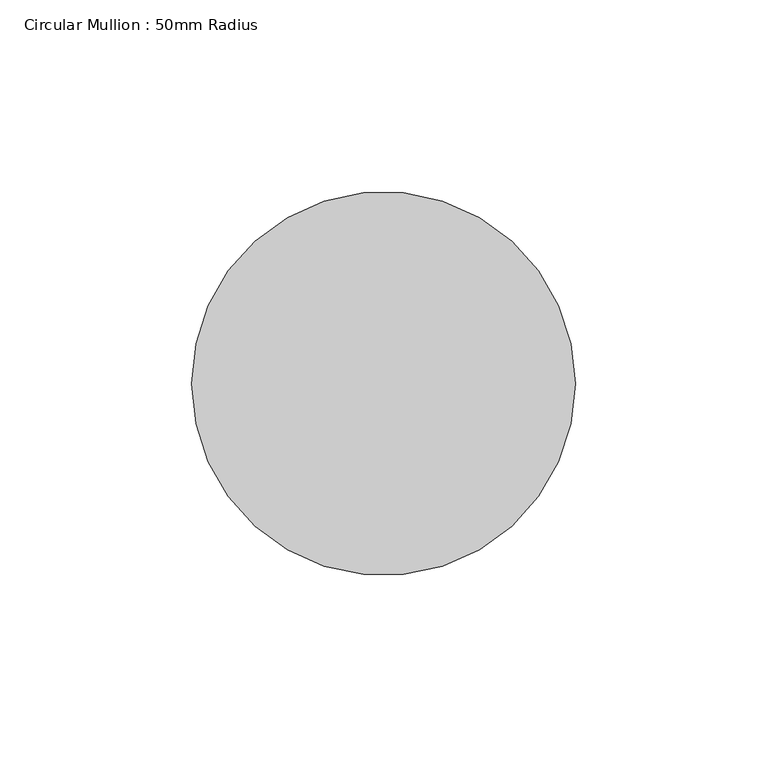
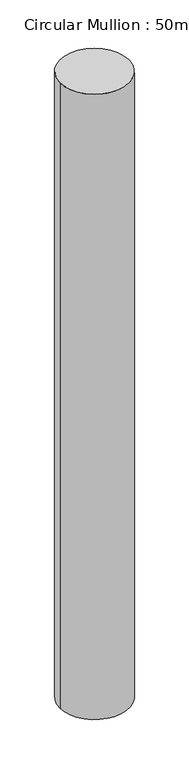
"""IFC4 building model written with IfcOpenShell, lengths in millimetres: member geometry, Circular Mullion : 50mm Radius."""

import ifcopenshell
import ifcopenshell.guid

model = None  # the IFC model being written
_history = None  # IfcOwnerHistory: only IFC2X3 demands one
_inside = {}  # id of a spatial element -> (the spatial element, [elements in it])
_under = {}  # id of a project, library or spatial element -> (it, [spatial elements below it])
_declared = {}  # id of a project -> (the project, [libraries it declares])
_typed = {}  # id of a type object -> (the type object, [elements of that type])
_made_of = {}  # id of a material, layer set ... -> (it, [elements and type objects made of it])


def new_model(schema):
    """Start an empty IFC model of exactly this schema.

    Asked for "IFC4X3", IfcOpenShell would pick the latest addendum, in which some entities
    have other attributes; the version numbers below select the first issue.
    IFC2X3 requires an IfcOwnerHistory on every rooted entity: one is made here for all.
    """
    global model, _history
    if schema == "IFC4X3":
        model = ifcopenshell.file(schema_version=(4, 3, 0, 0))
    else:
        model = ifcopenshell.file(schema=schema)
    _inside.clear()
    _under.clear()
    _declared.clear()
    _typed.clear()
    _made_of.clear()
    _history = None
    if model.schema == "IFC2X3":
        org = make("IfcOrganization", Name="unknown")
        user = make(
            "IfcPersonAndOrganization",
            ThePerson=make("IfcPerson", FamilyName="unknown"),
            TheOrganization=org,
        )
        app = make(
            "IfcApplication",
            ApplicationDeveloper=org,
            Version="unknown",
            ApplicationFullName="unknown",
            ApplicationIdentifier="unknown",
        )
        _history = make(
            "IfcOwnerHistory",
            OwningUser=user,
            OwningApplication=app,
            ChangeAction="ADDED",
            CreationDate=0,
        )
    return model


def make(cls, **values):
    """One entity of the class cls with the attributes given. An attribute that is None is left unset."""
    return model.create_entity(
        cls, **{name: value for name, value in values.items() if value is not None}
    )


def rooted(cls, **values):
    """An entity with a GlobalId (a new one), such as an element, a storey or a relation."""
    return make(cls, GlobalId=ifcopenshell.guid.new(), OwnerHistory=_history, **values)


def si_unit(unit_type, name, prefix=None):
    """IfcSIUnit, for example si_unit("LENGTHUNIT", "METRE", prefix="MILLI")."""
    return make("IfcSIUnit", UnitType=unit_type, Prefix=prefix, Name=name)


def assignment(units):
    """IfcUnitAssignment: the units of a project."""
    return None if units is None else make("IfcUnitAssignment", Units=units)


def point(xyz):
    """IfcCartesianPoint."""
    return None if xyz is None else make("IfcCartesianPoint", Coordinates=xyz)


def direction(xyz):
    """IfcDirection."""
    return None if xyz is None else make("IfcDirection", DirectionRatios=xyz)


def frame(location, z_axis=None, x_axis=None):
    """IfcAxis2Placement3D, a coordinate frame: its origin and axes. An axis left out is left unset."""
    return make(
        "IfcAxis2Placement3D",
        Location=point(location),
        Axis=direction(z_axis),
        RefDirection=direction(x_axis),
    )


def frame_2d(location, x_axis=None):
    """IfcAxis2Placement2D, a coordinate frame in the plane: its origin and x axis."""
    return make(
        "IfcAxis2Placement2D", Location=point(location), RefDirection=direction(x_axis)
    )


def origin():
    """The frame at (0, 0, 0) with its axes left unset."""
    return frame((0.0, 0.0, 0.0))


def origin_2d():
    """The frame at (0, 0) in the plane with its x axis left unset."""
    return frame_2d((0.0, 0.0))


def place(relative_to, where):
    """IfcLocalPlacement: puts the frame where relative to a parent placement (None: the world)."""
    return make(
        "IfcLocalPlacement", PlacementRelTo=relative_to, RelativePlacement=where
    )


def context(
    kind, dimensions, precision=None, world=None, true_north=None, identifier=None
):
    """IfcGeometricRepresentationContext, for example the 3D "Model" context."""
    return make(
        "IfcGeometricRepresentationContext",
        ContextIdentifier=identifier,
        ContextType=kind,
        CoordinateSpaceDimension=dimensions,
        Precision=precision,
        WorldCoordinateSystem=world,
        TrueNorth=true_north,
    )


def project(units=None, contexts=None):
    """IfcProject with its units and contexts."""
    return rooted(
        "IfcProject",
        Name="project",
        RepresentationContexts=contexts,
        UnitsInContext=assignment(units),
    )


def spatial(cls, under=None, at=None, **own):
    """A site, building, storey or space (cls), placed at a placement, below another one or the project."""
    s = rooted(cls, ObjectPlacement=at, **own)
    if under is not None:
        _under.setdefault(under.id(), (under, []))[1].append(s)
    return s


def circle_curve(where, radius):
    """IfcCircle in the frame where."""
    return make("IfcCircle", Position=where, Radius=radius)


def trimmed(basis, trim1, trim2, sense, master):
    """IfcTrimmedCurve: the piece of a basis curve between two trims."""
    return make(
        "IfcTrimmedCurve",
        BasisCurve=basis,
        Trim1=trim1,
        Trim2=trim2,
        SenseAgreement=sense,
        MasterRepresentation=master,
    )


def segment(curve, same_sense, transition):
    """IfcCompositeCurveSegment."""
    return make(
        "IfcCompositeCurveSegment",
        Transition=transition,
        SameSense=same_sense,
        ParentCurve=curve,
    )


def composite_curve(segments, self_intersect=None):
    """IfcCompositeCurve: segments joined end to end."""
    return make("IfcCompositeCurve", Segments=segments, SelfIntersect=self_intersect)


def outline(outer, holes=None, kind="AREA"):
    """IfcArbitraryClosedProfileDef: a profile drawn as a closed curve; with holes, ...WithVoids."""
    if holes is None:
        return make("IfcArbitraryClosedProfileDef", ProfileType=kind, OuterCurve=outer)
    return make(
        "IfcArbitraryProfileDefWithVoids",
        ProfileType=kind,
        OuterCurve=outer,
        InnerCurves=holes,
    )


def extrude(swept, where, along, depth):
    """IfcExtrudedAreaSolid: the profile swept, set in the frame where, extruded along a direction by depth."""
    return make(
        "IfcExtrudedAreaSolid",
        SweptArea=swept,
        Position=where,
        ExtrudedDirection=direction(along),
        Depth=depth,
    )


def shape(context_of_items, identifier, shape_type, items):
    """IfcShapeRepresentation: the items that make up one representation, for example the "Body"."""
    return make(
        "IfcShapeRepresentation",
        ContextOfItems=context_of_items,
        RepresentationIdentifier=identifier,
        RepresentationType=shape_type,
        Items=items,
    )


def source(mapping_origin, context_of_items, identifier, shape_type, items):
    """IfcRepresentationMap: a shape defined once, which mapped items show again and again."""
    return make(
        "IfcRepresentationMap",
        MappingOrigin=mapping_origin,
        MappedRepresentation=shape(context_of_items, identifier, shape_type, items),
    )


def transform(
    local_origin,
    x_axis=None,
    y_axis=None,
    z_axis=None,
    scale=None,
    scale2=None,
    scale3=None,
    uniform=True,
):
    """IfcCartesianTransformationOperator3D, or its non-uniform kind. x_axis, y_axis, z_axis: its Axis1, 2, 3."""
    if uniform:
        return make(
            "IfcCartesianTransformationOperator3D",
            Axis1=direction(x_axis),
            Axis2=direction(y_axis),
            LocalOrigin=point(local_origin),
            Scale=scale,
            Axis3=direction(z_axis),
        )
    return make(
        "IfcCartesianTransformationOperator3DnonUniform",
        Axis1=direction(x_axis),
        Axis2=direction(y_axis),
        LocalOrigin=point(local_origin),
        Scale=scale,
        Axis3=direction(z_axis),
        Scale2=scale2,
        Scale3=scale3,
    )


def mapped(mapping_source, mapping_target):
    """IfcMappedItem: shows the shape of a source again, moved by a transform."""
    return make(
        "IfcMappedItem", MappingSource=mapping_source, MappingTarget=mapping_target
    )


def made_of(thing, what):
    """Note that an element or type object is made of a material, layer set ...; save() writes the relation."""
    if what is not None:
        _made_of.setdefault(what.id(), (what, []))[1].append(thing)
    return thing


def element(
    cls,
    number,
    at=None,
    inside=None,
    cuts=None,
    type_object=None,
    material=None,
    context=None,
    identifier="Body",
    shape_type=None,
    held_by="IfcProductDefinitionShape",
    body=None,
    shapes=None,
    **own,
):
    """One element of the class cls, such as IfcWall. Its Tag is "e" and its number.

    at: its placement. inside: the storey or other place that contains it. cuts: it is an
    opening in that element (IfcRelVoidsElement). A single representation is given by context,
    identifier, shape_type and body (its items); several are given by shapes. held_by: the class
    of the entity that holds the representations. save() writes the other relations.
    """
    e = rooted(cls, Tag="e%d" % number, ObjectPlacement=at, **own)
    if body is not None:
        shapes = [shape(context, identifier, shape_type, body)]
    if shapes is not None:
        e.Representation = make(held_by, Representations=shapes)
    if inside is not None:
        _inside.setdefault(inside.id(), (inside, []))[1].append(e)
    if cuts is not None:
        rooted(
            "IfcRelVoidsElement", RelatingBuildingElement=cuts, RelatedOpeningElement=e
        )
    if type_object is not None:
        _typed.setdefault(type_object.id(), (type_object, []))[1].append(e)
    return made_of(e, material)


def aggregate(whole, parts):
    """IfcRelAggregates: a whole, such as a stair, and the parts it consists of."""
    return rooted("IfcRelAggregates", RelatingObject=whole, RelatedObjects=parts)


def save(model, path):
    """Write the relations noted so far, then the file.

    IfcRelAggregates (storeys below a building ...), IfcRelContainedInSpatialStructure (elements
    in a storey), IfcRelDefinesByType, IfcRelAssociatesMaterial and IfcRelDeclares: one each for
    every whole, place, type object, material and project.
    """
    for whole, parts in _under.values():
        aggregate(whole, parts)
    for where, things in _inside.values():
        rooted(
            "IfcRelContainedInSpatialStructure",
            RelatedElements=things,
            RelatingStructure=where,
        )
    for kind, things in _typed.values():
        rooted("IfcRelDefinesByType", RelatedObjects=things, RelatingType=kind)
    for what, things in _made_of.values():
        rooted("IfcRelAssociatesMaterial", RelatedObjects=things, RelatingMaterial=what)
    for by, libraries in _declared.values():
        rooted("IfcRelDeclares", RelatingContext=by, RelatedDefinitions=libraries)
    model.write(path)


def circular_mullion_50mm_radius_cafa9232(model_context):
    return source(origin(), model_context, "Body", "SweptSolid", [
        extrude(outline(composite_curve([segment(trimmed(circle_curve(origin_2d(), 50.0), [point((50.0, 0.0))], [point((-50.0, 0.0))], False, "CARTESIAN"), True, "CONTINUOUS"), segment(trimmed(circle_curve(origin_2d(), 50.0), [point((-50.0, 0.0))], [point((50.0, 0.0))], False, "CARTESIAN"), True, "CONTINUOUS")], self_intersect=False)), frame((0.0, 0.0, -953.7925357), z_axis=(0.0, 0.0, 1.0), x_axis=(1.0, 0.0, 0.0)), (0.0, 0.0, 1.0), 953.7925357),
    ])


if __name__ == "__main__":
    model = new_model("IFC4")
    model_context = context("Model", 3, world=origin())
    ifc_project = project(units=[si_unit("LENGTHUNIT", "METRE", prefix="MILLI")], contexts=[model_context])
    site = spatial("IfcSite", under=ifc_project)
    building = spatial("IfcBuilding", under=site)
    placement = place(None, origin())
    circular_mullion_50mm_radius_shape = circular_mullion_50mm_radius_cafa9232(model_context)
    element("IfcMember", 1, ObjectType="Circular Mullion : 50mm Radius", at=placement, inside=building, context=model_context, shape_type="MappedRepresentation", body=[
        mapped(circular_mullion_50mm_radius_shape, transform((0.0, 0.0, 0.0), x_axis=(1.0, 0.0, 0.0), y_axis=(0.0, 1.0, 0.0), z_axis=(0.0, 0.0, 1.0))),
    ])
    save(model, "model.ifc")

# Revit data of these elements
# Type "Circular Mullion : 50mm Radius"
#   built-in parameter 1007350 = 0.164042 (stored number, unit not read)
# Element 1 (IfcMember, "Circular Mullion : 50mm Radius")
#   Materials on its faces: "Aluminium"
# Materials
#   "Aluminium": class "Metal", colour RGB 247 247 247, transparency 0, Description = "Aluminium 6061", Cost = 0
